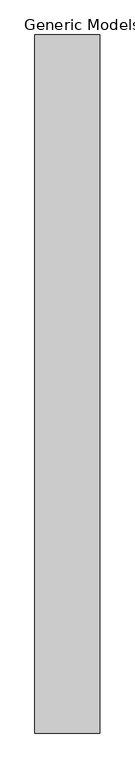
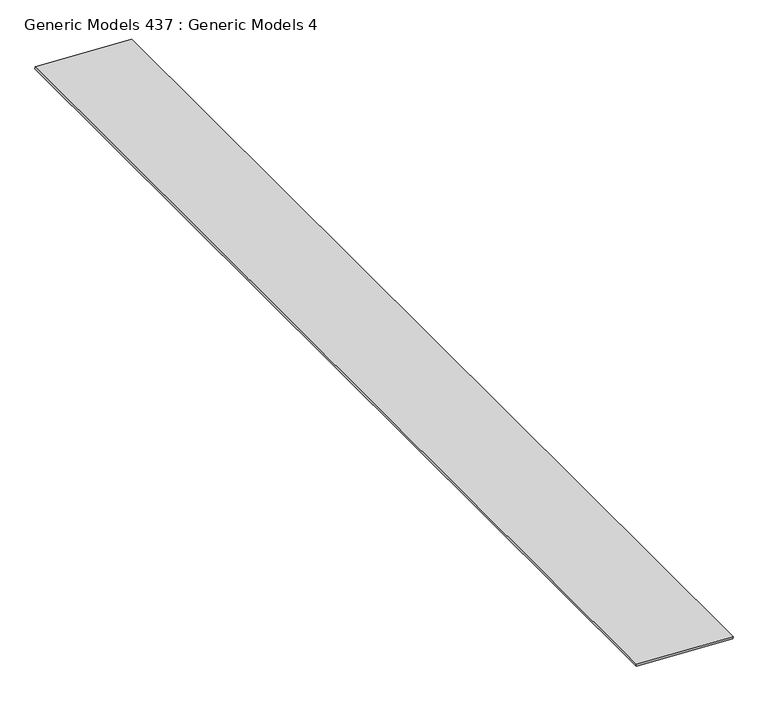
"""IFC4 building model written with IfcOpenShell, lengths in millimetres: proxy geometry, Generic Models 437 : Generic Models 4."""

from ifc_helpers import new_model, si_unit, frame, origin, place, context, project, spatial, polyline, outline, extrude, source, transform, mapped, element, save


def generic_models_437_generic_models_4_cee23a1c(model_context):
    return source(origin(), model_context, "Body", "SweptSolid", [
        extrude(outline(polyline([(0.0, -1165.74819), (0.0, 0.0), (12547.6, 0.0), (12547.6, -1165.74819), (0.0, -1165.74819)])), frame((8574.8779329, -5493.3230338, 123577.4126988), z_axis=(0.047039883592958916, 0.0, 0.9988930119645251), x_axis=(0.0, 1.0, 0.0)), (0.0, 0.0, 1.0), 25.4),
    ])


if __name__ == "__main__":
    model = new_model("IFC4")
    model_context = context("Model", 3, world=origin())
    ifc_project = project(units=[si_unit("LENGTHUNIT", "METRE", prefix="MILLI")], contexts=[model_context])
    site = spatial("IfcSite", under=ifc_project)
    building = spatial("IfcBuilding", under=site)
    placement = place(None, origin())
    generic_models_437_generic_models_4_shape = generic_models_437_generic_models_4_cee23a1c(model_context)
    element("IfcBuildingElementProxy", 1, Name="Generic Models 437 : Generic Models 4", ObjectType="Generic Models 437 : Generic Models 4", at=placement, inside=building, context=model_context, shape_type="MappedRepresentation", body=[
        mapped(generic_models_437_generic_models_4_shape, transform((0.0, 0.0, 0.0), x_axis=(1.0, 0.0, 0.0), y_axis=(0.0, 1.0, 0.0), z_axis=(0.0, 0.0, 1.0))),
    ])
    save(model, "model.ifc")

# Revit data of these elements
# Element 1 (IfcBuildingElementProxy, "Generic Models 437 : Generic Models 4")
#   Materials on its faces: "_1\" BEDDING SAND"
# Materials
#   "_1\" BEDDING SAND": class "Generic", colour RGB 245 226 173, transparency 0, Cost = 0
